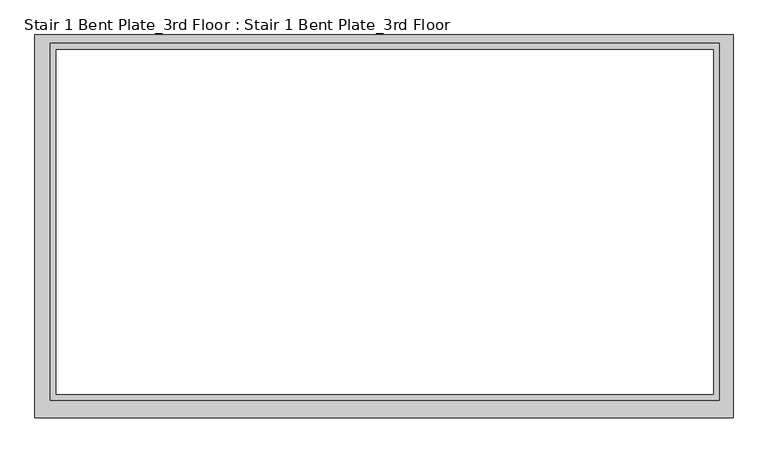
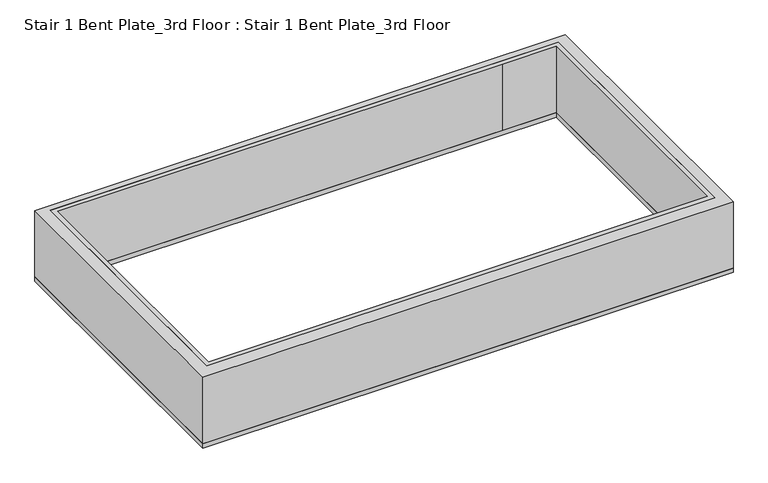
"""IFC4 building model written with IfcOpenShell, lengths in millimetres: proxy geometry, Stair 1 Bent Plate_3rd Floor : Stair 1 Bent Plate_3rd Floor."""

import ifcopenshell
import ifcopenshell.guid

model = None  # the IFC model being written
_history = None  # IfcOwnerHistory: only IFC2X3 demands one
_inside = {}  # id of a spatial element -> (the spatial element, [elements in it])
_under = {}  # id of a project, library or spatial element -> (it, [spatial elements below it])
_declared = {}  # id of a project -> (the project, [libraries it declares])
_typed = {}  # id of a type object -> (the type object, [elements of that type])
_made_of = {}  # id of a material, layer set ... -> (it, [elements and type objects made of it])


def new_model(schema):
    """Start an empty IFC model of exactly this schema.

    Asked for "IFC4X3", IfcOpenShell would pick the latest addendum, in which some entities
    have other attributes; the version numbers below select the first issue.
    IFC2X3 requires an IfcOwnerHistory on every rooted entity: one is made here for all.
    """
    global model, _history
    if schema == "IFC4X3":
        model = ifcopenshell.file(schema_version=(4, 3, 0, 0))
    else:
        model = ifcopenshell.file(schema=schema)
    _inside.clear()
    _under.clear()
    _declared.clear()
    _typed.clear()
    _made_of.clear()
    _history = None
    if model.schema == "IFC2X3":
        org = make("IfcOrganization", Name="unknown")
        user = make(
            "IfcPersonAndOrganization",
            ThePerson=make("IfcPerson", FamilyName="unknown"),
            TheOrganization=org,
        )
        app = make(
            "IfcApplication",
            ApplicationDeveloper=org,
            Version="unknown",
            ApplicationFullName="unknown",
            ApplicationIdentifier="unknown",
        )
        _history = make(
            "IfcOwnerHistory",
            OwningUser=user,
            OwningApplication=app,
            ChangeAction="ADDED",
            CreationDate=0,
        )
    return model


def make(cls, **values):
    """One entity of the class cls with the attributes given. An attribute that is None is left unset."""
    return model.create_entity(
        cls, **{name: value for name, value in values.items() if value is not None}
    )


def rooted(cls, **values):
    """An entity with a GlobalId (a new one), such as an element, a storey or a relation."""
    return make(cls, GlobalId=ifcopenshell.guid.new(), OwnerHistory=_history, **values)


def si_unit(unit_type, name, prefix=None):
    """IfcSIUnit, for example si_unit("LENGTHUNIT", "METRE", prefix="MILLI")."""
    return make("IfcSIUnit", UnitType=unit_type, Prefix=prefix, Name=name)


def assignment(units):
    """IfcUnitAssignment: the units of a project."""
    return None if units is None else make("IfcUnitAssignment", Units=units)


def point(xyz):
    """IfcCartesianPoint."""
    return None if xyz is None else make("IfcCartesianPoint", Coordinates=xyz)


def direction(xyz):
    """IfcDirection."""
    return None if xyz is None else make("IfcDirection", DirectionRatios=xyz)


def frame(location, z_axis=None, x_axis=None):
    """IfcAxis2Placement3D, a coordinate frame: its origin and axes. An axis left out is left unset."""
    return make(
        "IfcAxis2Placement3D",
        Location=point(location),
        Axis=direction(z_axis),
        RefDirection=direction(x_axis),
    )


def origin():
    """The frame at (0, 0, 0) with its axes left unset."""
    return frame((0.0, 0.0, 0.0))


def origin_with_axes():
    """The frame at (0, 0, 0) with the z axis (0, 0, 1) and the x axis (1, 0, 0) written out."""
    return frame((0.0, 0.0, 0.0), z_axis=(0.0, 0.0, 1.0), x_axis=(1.0, 0.0, 0.0))


def place(relative_to, where):
    """IfcLocalPlacement: puts the frame where relative to a parent placement (None: the world)."""
    return make(
        "IfcLocalPlacement", PlacementRelTo=relative_to, RelativePlacement=where
    )


def context(
    kind, dimensions, precision=None, world=None, true_north=None, identifier=None
):
    """IfcGeometricRepresentationContext, for example the 3D "Model" context."""
    return make(
        "IfcGeometricRepresentationContext",
        ContextIdentifier=identifier,
        ContextType=kind,
        CoordinateSpaceDimension=dimensions,
        Precision=precision,
        WorldCoordinateSystem=world,
        TrueNorth=true_north,
    )


def project(units=None, contexts=None):
    """IfcProject with its units and contexts."""
    return rooted(
        "IfcProject",
        Name="project",
        RepresentationContexts=contexts,
        UnitsInContext=assignment(units),
    )


def spatial(cls, under=None, at=None, **own):
    """A site, building, storey or space (cls), placed at a placement, below another one or the project."""
    s = rooted(cls, ObjectPlacement=at, **own)
    if under is not None:
        _under.setdefault(under.id(), (under, []))[1].append(s)
    return s


def polyline(points):
    """IfcPolyline through the points."""
    return make("IfcPolyline", Points=[point(p) for p in points])


def outline(outer, holes=None, kind="AREA"):
    """IfcArbitraryClosedProfileDef: a profile drawn as a closed curve; with holes, ...WithVoids."""
    if holes is None:
        return make("IfcArbitraryClosedProfileDef", ProfileType=kind, OuterCurve=outer)
    return make(
        "IfcArbitraryProfileDefWithVoids",
        ProfileType=kind,
        OuterCurve=outer,
        InnerCurves=holes,
    )


def extrude(swept, where, along, depth):
    """IfcExtrudedAreaSolid: the profile swept, set in the frame where, extruded along a direction by depth."""
    return make(
        "IfcExtrudedAreaSolid",
        SweptArea=swept,
        Position=where,
        ExtrudedDirection=direction(along),
        Depth=depth,
    )


def shape(context_of_items, identifier, shape_type, items):
    """IfcShapeRepresentation: the items that make up one representation, for example the "Body"."""
    return make(
        "IfcShapeRepresentation",
        ContextOfItems=context_of_items,
        RepresentationIdentifier=identifier,
        RepresentationType=shape_type,
        Items=items,
    )


def source(mapping_origin, context_of_items, identifier, shape_type, items):
    """IfcRepresentationMap: a shape defined once, which mapped items show again and again."""
    return make(
        "IfcRepresentationMap",
        MappingOrigin=mapping_origin,
        MappedRepresentation=shape(context_of_items, identifier, shape_type, items),
    )


def transform(
    local_origin,
    x_axis=None,
    y_axis=None,
    z_axis=None,
    scale=None,
    scale2=None,
    scale3=None,
    uniform=True,
):
    """IfcCartesianTransformationOperator3D, or its non-uniform kind. x_axis, y_axis, z_axis: its Axis1, 2, 3."""
    if uniform:
        return make(
            "IfcCartesianTransformationOperator3D",
            Axis1=direction(x_axis),
            Axis2=direction(y_axis),
            LocalOrigin=point(local_origin),
            Scale=scale,
            Axis3=direction(z_axis),
        )
    return make(
        "IfcCartesianTransformationOperator3DnonUniform",
        Axis1=direction(x_axis),
        Axis2=direction(y_axis),
        LocalOrigin=point(local_origin),
        Scale=scale,
        Axis3=direction(z_axis),
        Scale2=scale2,
        Scale3=scale3,
    )


def mapped(mapping_source, mapping_target):
    """IfcMappedItem: shows the shape of a source again, moved by a transform."""
    return make(
        "IfcMappedItem", MappingSource=mapping_source, MappingTarget=mapping_target
    )


def made_of(thing, what):
    """Note that an element or type object is made of a material, layer set ...; save() writes the relation."""
    if what is not None:
        _made_of.setdefault(what.id(), (what, []))[1].append(thing)
    return thing


def element(
    cls,
    number,
    at=None,
    inside=None,
    cuts=None,
    type_object=None,
    material=None,
    context=None,
    identifier="Body",
    shape_type=None,
    held_by="IfcProductDefinitionShape",
    body=None,
    shapes=None,
    **own,
):
    """One element of the class cls, such as IfcWall. Its Tag is "e" and its number.

    at: its placement. inside: the storey or other place that contains it. cuts: it is an
    opening in that element (IfcRelVoidsElement). A single representation is given by context,
    identifier, shape_type and body (its items); several are given by shapes. held_by: the class
    of the entity that holds the representations. save() writes the other relations.
    """
    e = rooted(cls, Tag="e%d" % number, ObjectPlacement=at, **own)
    if body is not None:
        shapes = [shape(context, identifier, shape_type, body)]
    if shapes is not None:
        e.Representation = make(held_by, Representations=shapes)
    if inside is not None:
        _inside.setdefault(inside.id(), (inside, []))[1].append(e)
    if cuts is not None:
        rooted(
            "IfcRelVoidsElement", RelatingBuildingElement=cuts, RelatedOpeningElement=e
        )
    if type_object is not None:
        _typed.setdefault(type_object.id(), (type_object, []))[1].append(e)
    return made_of(e, material)


def aggregate(whole, parts):
    """IfcRelAggregates: a whole, such as a stair, and the parts it consists of."""
    return rooted("IfcRelAggregates", RelatingObject=whole, RelatedObjects=parts)


def save(model, path):
    """Write the relations noted so far, then the file.

    IfcRelAggregates (storeys below a building ...), IfcRelContainedInSpatialStructure (elements
    in a storey), IfcRelDefinesByType, IfcRelAssociatesMaterial and IfcRelDeclares: one each for
    every whole, place, type object, material and project.
    """
    for whole, parts in _under.values():
        aggregate(whole, parts)
    for where, things in _inside.values():
        rooted(
            "IfcRelContainedInSpatialStructure",
            RelatedElements=things,
            RelatingStructure=where,
        )
    for kind, things in _typed.values():
        rooted("IfcRelDefinesByType", RelatedObjects=things, RelatingType=kind)
    for what, things in _made_of.values():
        rooted("IfcRelAssociatesMaterial", RelatedObjects=things, RelatingMaterial=what)
    for by, libraries in _declared.values():
        rooted("IfcRelDeclares", RelatingContext=by, RelatedDefinitions=libraries)
    model.write(path)


def stair_1_bent_plate_3rd_floor_stair_1_bent_plate_3rd_floor_ed8e0977(model_context):
    return source(origin(), model_context, "Body", "SweptSolid", [
        extrude(outline(polyline([(-279.4, -750.8875), (-279.4, 39.7358273), (1162.05, 39.7358273), (1162.05, -750.8875), (-279.4, -750.8875)]), holes=[polyline([(1133.475, 22.225), (-247.65, 22.225), (-247.65, -714.375), (1133.475, -714.375), (1133.475, 22.225)])]), frame((0.0, 0.0, 12.7), z_axis=(0.0, 0.0, 1.0), x_axis=(1.0, 0.0, 0.0)), (0.0, 0.0, 1.0), 190.5),
        extrude(outline(polyline([(1162.05, -750.8875), (-279.4, -750.8875), (-279.4, 39.7358273), (1162.05, 39.7358273), (1162.05, -750.8875)]), holes=[polyline([(-234.95, 9.525), (-234.95, -701.675), (1120.775, -701.675), (1120.775, 9.525), (-234.95, 9.525)])]), origin_with_axes(), (0.0, 0.0, 1.0), 12.7),
        extrude(outline(polyline([(1133.475, 22.225), (1133.475, -714.375), (-247.65, -714.375), (-247.65, 22.225), (1133.475, 22.225)]), holes=[polyline([(-234.95, -701.675), (1120.775, -701.675), (1120.775, 9.525), (974.725, 9.525), (-234.95, 9.525), (-234.95, -190.5), (-234.95, -701.675)])]), origin_with_axes(), (0.0, 0.0, 1.0), 203.2),
    ])


if __name__ == "__main__":
    model = new_model("IFC4")
    model_context = context("Model", 3, world=origin())
    ifc_project = project(units=[si_unit("LENGTHUNIT", "METRE", prefix="MILLI")], contexts=[model_context])
    site = spatial("IfcSite", under=ifc_project)
    building = spatial("IfcBuilding", under=site)
    placement = place(None, origin())
    stair_1_bent_plate_3rd_floor_stair_1_bent_plate_3rd_floor_shape = stair_1_bent_plate_3rd_floor_stair_1_bent_plate_3rd_floor_ed8e0977(model_context)
    element("IfcBuildingElementProxy", 1, Name="Stair 1 Bent Plate_3rd Floor : Stair 1 Bent Plate_3rd Floor", ObjectType="Stair 1 Bent Plate_3rd Floor : Stair 1 Bent Plate_3rd Floor", at=placement, inside=building, context=model_context, shape_type="MappedRepresentation", body=[
        mapped(stair_1_bent_plate_3rd_floor_stair_1_bent_plate_3rd_floor_shape, transform((0.0, 0.0, 0.0), x_axis=(1.0, 0.0, 0.0), y_axis=(0.0, 1.0, 0.0), z_axis=(0.0, 0.0, 1.0))),
    ])
    save(model, "model.ifc")

# Revit data of these elements
# Element 1 (IfcBuildingElementProxy, "Stair 1 Bent Plate_3rd Floor : Stair 1 Bent Plate_3rd Floor")
#   Materials on its faces: "Concrete Infill"
# Materials
#   "Concrete Infill": class "Generic", colour RGB 0 255 0, transparency 0, Cost = 0
